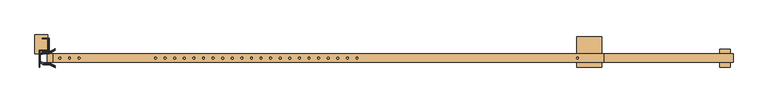
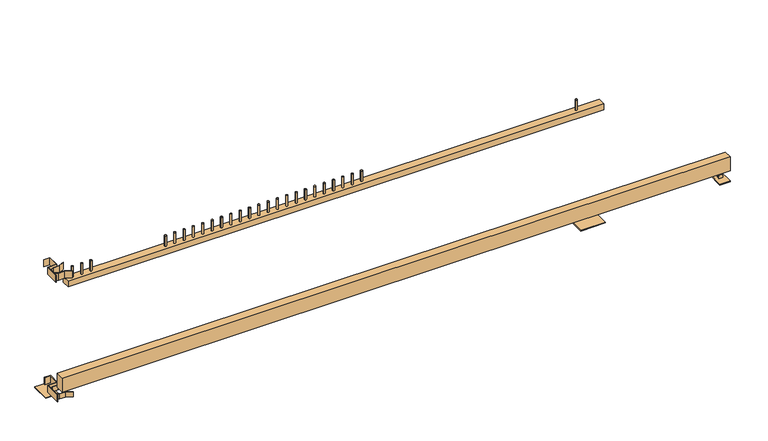
"""IFC4 building model written with IfcOpenShell, lengths in millimetres: door geometry, NLRS_90_DO_UN_schuifpoort met spijlen_gen_rsf : schuifpoort automatisch bxh 7000x1800-NP."""

import ifcopenshell
import ifcopenshell.guid

model = None  # the IFC model being written
_history = None  # IfcOwnerHistory: only IFC2X3 demands one
_inside = {}  # id of a spatial element -> (the spatial element, [elements in it])
_under = {}  # id of a project, library or spatial element -> (it, [spatial elements below it])
_declared = {}  # id of a project -> (the project, [libraries it declares])
_typed = {}  # id of a type object -> (the type object, [elements of that type])
_made_of = {}  # id of a material, layer set ... -> (it, [elements and type objects made of it])


def new_model(schema):
    """Start an empty IFC model of exactly this schema.

    Asked for "IFC4X3", IfcOpenShell would pick the latest addendum, in which some entities
    have other attributes; the version numbers below select the first issue.
    IFC2X3 requires an IfcOwnerHistory on every rooted entity: one is made here for all.
    """
    global model, _history
    if schema == "IFC4X3":
        model = ifcopenshell.file(schema_version=(4, 3, 0, 0))
    else:
        model = ifcopenshell.file(schema=schema)
    _inside.clear()
    _under.clear()
    _declared.clear()
    _typed.clear()
    _made_of.clear()
    _history = None
    if model.schema == "IFC2X3":
        org = make("IfcOrganization", Name="unknown")
        user = make(
            "IfcPersonAndOrganization",
            ThePerson=make("IfcPerson", FamilyName="unknown"),
            TheOrganization=org,
        )
        app = make(
            "IfcApplication",
            ApplicationDeveloper=org,
            Version="unknown",
            ApplicationFullName="unknown",
            ApplicationIdentifier="unknown",
        )
        _history = make(
            "IfcOwnerHistory",
            OwningUser=user,
            OwningApplication=app,
            ChangeAction="ADDED",
            CreationDate=0,
        )
    return model


def make(cls, **values):
    """One entity of the class cls with the attributes given. An attribute that is None is left unset."""
    return model.create_entity(
        cls, **{name: value for name, value in values.items() if value is not None}
    )


def rooted(cls, **values):
    """An entity with a GlobalId (a new one), such as an element, a storey or a relation."""
    return make(cls, GlobalId=ifcopenshell.guid.new(), OwnerHistory=_history, **values)


def si_unit(unit_type, name, prefix=None):
    """IfcSIUnit, for example si_unit("LENGTHUNIT", "METRE", prefix="MILLI")."""
    return make("IfcSIUnit", UnitType=unit_type, Prefix=prefix, Name=name)


def assignment(units):
    """IfcUnitAssignment: the units of a project."""
    return None if units is None else make("IfcUnitAssignment", Units=units)


def point(xyz):
    """IfcCartesianPoint."""
    return None if xyz is None else make("IfcCartesianPoint", Coordinates=xyz)


def direction(xyz):
    """IfcDirection."""
    return None if xyz is None else make("IfcDirection", DirectionRatios=xyz)


def frame(location, z_axis=None, x_axis=None):
    """IfcAxis2Placement3D, a coordinate frame: its origin and axes. An axis left out is left unset."""
    return make(
        "IfcAxis2Placement3D",
        Location=point(location),
        Axis=direction(z_axis),
        RefDirection=direction(x_axis),
    )


def frame_2d(location, x_axis=None):
    """IfcAxis2Placement2D, a coordinate frame in the plane: its origin and x axis."""
    return make(
        "IfcAxis2Placement2D", Location=point(location), RefDirection=direction(x_axis)
    )


def origin():
    """The frame at (0, 0, 0) with its axes left unset."""
    return frame((0.0, 0.0, 0.0))


def origin_with_axes():
    """The frame at (0, 0, 0) with the z axis (0, 0, 1) and the x axis (1, 0, 0) written out."""
    return frame((0.0, 0.0, 0.0), z_axis=(0.0, 0.0, 1.0), x_axis=(1.0, 0.0, 0.0))


def place(relative_to, where):
    """IfcLocalPlacement: puts the frame where relative to a parent placement (None: the world)."""
    return make(
        "IfcLocalPlacement", PlacementRelTo=relative_to, RelativePlacement=where
    )


def context(
    kind, dimensions, precision=None, world=None, true_north=None, identifier=None
):
    """IfcGeometricRepresentationContext, for example the 3D "Model" context."""
    return make(
        "IfcGeometricRepresentationContext",
        ContextIdentifier=identifier,
        ContextType=kind,
        CoordinateSpaceDimension=dimensions,
        Precision=precision,
        WorldCoordinateSystem=world,
        TrueNorth=true_north,
    )


def project(units=None, contexts=None):
    """IfcProject with its units and contexts."""
    return rooted(
        "IfcProject",
        Name="project",
        RepresentationContexts=contexts,
        UnitsInContext=assignment(units),
    )


def spatial(cls, under=None, at=None, **own):
    """A site, building, storey or space (cls), placed at a placement, below another one or the project."""
    s = rooted(cls, ObjectPlacement=at, **own)
    if under is not None:
        _under.setdefault(under.id(), (under, []))[1].append(s)
    return s


def polyline(points):
    """IfcPolyline through the points."""
    return make("IfcPolyline", Points=[point(p) for p in points])


def circle_curve(where, radius):
    """IfcCircle in the frame where."""
    return make("IfcCircle", Position=where, Radius=radius)


def trimmed(basis, trim1, trim2, sense, master):
    """IfcTrimmedCurve: the piece of a basis curve between two trims."""
    return make(
        "IfcTrimmedCurve",
        BasisCurve=basis,
        Trim1=trim1,
        Trim2=trim2,
        SenseAgreement=sense,
        MasterRepresentation=master,
    )


def segment(curve, same_sense, transition):
    """IfcCompositeCurveSegment."""
    return make(
        "IfcCompositeCurveSegment",
        Transition=transition,
        SameSense=same_sense,
        ParentCurve=curve,
    )


def composite_curve(segments, self_intersect=None):
    """IfcCompositeCurve: segments joined end to end."""
    return make("IfcCompositeCurve", Segments=segments, SelfIntersect=self_intersect)


def outline(outer, holes=None, kind="AREA"):
    """IfcArbitraryClosedProfileDef: a profile drawn as a closed curve; with holes, ...WithVoids."""
    if holes is None:
        return make("IfcArbitraryClosedProfileDef", ProfileType=kind, OuterCurve=outer)
    return make(
        "IfcArbitraryProfileDefWithVoids",
        ProfileType=kind,
        OuterCurve=outer,
        InnerCurves=holes,
    )


def extrude(swept, where, along, depth):
    """IfcExtrudedAreaSolid: the profile swept, set in the frame where, extruded along a direction by depth."""
    return make(
        "IfcExtrudedAreaSolid",
        SweptArea=swept,
        Position=where,
        ExtrudedDirection=direction(along),
        Depth=depth,
    )


def shape(context_of_items, identifier, shape_type, items):
    """IfcShapeRepresentation: the items that make up one representation, for example the "Body"."""
    return make(
        "IfcShapeRepresentation",
        ContextOfItems=context_of_items,
        RepresentationIdentifier=identifier,
        RepresentationType=shape_type,
        Items=items,
    )


def source(mapping_origin, context_of_items, identifier, shape_type, items):
    """IfcRepresentationMap: a shape defined once, which mapped items show again and again."""
    return make(
        "IfcRepresentationMap",
        MappingOrigin=mapping_origin,
        MappedRepresentation=shape(context_of_items, identifier, shape_type, items),
    )


def transform(
    local_origin,
    x_axis=None,
    y_axis=None,
    z_axis=None,
    scale=None,
    scale2=None,
    scale3=None,
    uniform=True,
):
    """IfcCartesianTransformationOperator3D, or its non-uniform kind. x_axis, y_axis, z_axis: its Axis1, 2, 3."""
    if uniform:
        return make(
            "IfcCartesianTransformationOperator3D",
            Axis1=direction(x_axis),
            Axis2=direction(y_axis),
            LocalOrigin=point(local_origin),
            Scale=scale,
            Axis3=direction(z_axis),
        )
    return make(
        "IfcCartesianTransformationOperator3DnonUniform",
        Axis1=direction(x_axis),
        Axis2=direction(y_axis),
        LocalOrigin=point(local_origin),
        Scale=scale,
        Axis3=direction(z_axis),
        Scale2=scale2,
        Scale3=scale3,
    )


def mapped(mapping_source, mapping_target):
    """IfcMappedItem: shows the shape of a source again, moved by a transform."""
    return make(
        "IfcMappedItem", MappingSource=mapping_source, MappingTarget=mapping_target
    )


def made_of(thing, what):
    """Note that an element or type object is made of a material, layer set ...; save() writes the relation."""
    if what is not None:
        _made_of.setdefault(what.id(), (what, []))[1].append(thing)
    return thing


def element(
    cls,
    number,
    at=None,
    inside=None,
    cuts=None,
    type_object=None,
    material=None,
    context=None,
    identifier="Body",
    shape_type=None,
    held_by="IfcProductDefinitionShape",
    body=None,
    shapes=None,
    **own,
):
    """One element of the class cls, such as IfcWall. Its Tag is "e" and its number.

    at: its placement. inside: the storey or other place that contains it. cuts: it is an
    opening in that element (IfcRelVoidsElement). A single representation is given by context,
    identifier, shape_type and body (its items); several are given by shapes. held_by: the class
    of the entity that holds the representations. save() writes the other relations.
    """
    e = rooted(cls, Tag="e%d" % number, ObjectPlacement=at, **own)
    if body is not None:
        shapes = [shape(context, identifier, shape_type, body)]
    if shapes is not None:
        e.Representation = make(held_by, Representations=shapes)
    if inside is not None:
        _inside.setdefault(inside.id(), (inside, []))[1].append(e)
    if cuts is not None:
        rooted(
            "IfcRelVoidsElement", RelatingBuildingElement=cuts, RelatedOpeningElement=e
        )
    if type_object is not None:
        _typed.setdefault(type_object.id(), (type_object, []))[1].append(e)
    return made_of(e, material)


def aggregate(whole, parts):
    """IfcRelAggregates: a whole, such as a stair, and the parts it consists of."""
    return rooted("IfcRelAggregates", RelatingObject=whole, RelatedObjects=parts)


def save(model, path):
    """Write the relations noted so far, then the file.

    IfcRelAggregates (storeys below a building ...), IfcRelContainedInSpatialStructure (elements
    in a storey), IfcRelDefinesByType, IfcRelAssociatesMaterial and IfcRelDeclares: one each for
    every whole, place, type object, material and project.
    """
    for whole, parts in _under.values():
        aggregate(whole, parts)
    for where, things in _inside.values():
        rooted(
            "IfcRelContainedInSpatialStructure",
            RelatedElements=things,
            RelatingStructure=where,
        )
    for kind, things in _typed.values():
        rooted("IfcRelDefinesByType", RelatedObjects=things, RelatingType=kind)
    for what, things in _made_of.values():
        rooted("IfcRelAssociatesMaterial", RelatedObjects=things, RelatingMaterial=what)
    for by, libraries in _declared.values():
        rooted("IfcRelDeclares", RelatingContext=by, RelatedDefinitions=libraries)
    model.write(path)


def door_84a52a24(model_context):
    return source(origin(), model_context, "Body", "SweptSolid", [
        extrude(outline(composite_curve([segment(trimmed(circle_curve(frame_2d((-3115.5, 0.0)), 12.5), [point((-3103.0, 0.0))], [point((-3128.0, 0.0))], False, "CARTESIAN"), True, "CONTINUOUS"), segment(trimmed(circle_curve(frame_2d((-3115.5, 0.0)), 12.5), [point((-3128.0, 0.0))], [point((-3103.0, 0.0))], False, "CARTESIAN"), True, "CONTINUOUS")], self_intersect=False)), frame((0.0, 0.0, 1650.0), z_axis=(0.0, 0.0, 1.0), x_axis=(1.0, 0.0, 0.0)), (0.0, 0.0, 1.0), 150.0),
        extrude(outline(composite_curve([segment(trimmed(circle_curve(frame_2d((-3241.5, 0.0)), 12.5), [point((-3229.0, 0.0))], [point((-3254.0, 0.0))], False, "CARTESIAN"), True, "CONTINUOUS"), segment(trimmed(circle_curve(frame_2d((-3241.5, 0.0)), 12.5), [point((-3254.0, 0.0))], [point((-3229.0, 0.0))], False, "CARTESIAN"), True, "CONTINUOUS")], self_intersect=False)), frame((0.0, 0.0, 1650.0), z_axis=(0.0, 0.0, 1.0), x_axis=(1.0, 0.0, 0.0)), (0.0, 0.0, 1.0), 150.0),
        extrude(outline(composite_curve([segment(trimmed(circle_curve(frame_2d((-3367.5, 0.0)), 12.5), [point((-3355.0, 0.0))], [point((-3380.0, 0.0))], False, "CARTESIAN"), True, "CONTINUOUS"), segment(trimmed(circle_curve(frame_2d((-3367.5, 0.0)), 12.5), [point((-3380.0, 0.0))], [point((-3355.0, 0.0))], False, "CARTESIAN"), True, "CONTINUOUS")], self_intersect=False)), frame((0.0, 0.0, 1650.0), z_axis=(0.0, 0.0, 1.0), x_axis=(1.0, 0.0, 0.0)), (0.0, 0.0, 1.0), 150.0),
        extrude(outline(polyline([(3745.0, 280.5), (3745.0, -119.5), (3415.0, -119.5), (3415.0, 280.5), (3745.0, 280.5)])), origin_with_axes(), (0.0, 0.0, 1.0), 12.0),
        extrude(outline(composite_curve([segment(trimmed(circle_curve(frame_2d((3424.5, 0.0)), 12.5), [point((3437.0, 0.0))], [point((3412.0, 0.0))], False, "CARTESIAN"), True, "CONTINUOUS"), segment(trimmed(circle_curve(frame_2d((3424.5, 0.0)), 12.5), [point((3412.0, 0.0))], [point((3437.0, 0.0))], False, "CARTESIAN"), True, "CONTINUOUS")], self_intersect=False)), frame((0.0, 0.0, 1650.0), z_axis=(0.0, 0.0, 1.0), x_axis=(1.0, 0.0, 0.0)), (0.0, 0.0, 1.0), 150.0),
        extrude(outline(composite_curve([segment(trimmed(circle_curve(frame_2d((-727.5, 0.0)), 12.5), [point((-715.0, 0.0))], [point((-740.0, 0.0))], False, "CARTESIAN"), True, "CONTINUOUS"), segment(trimmed(circle_curve(frame_2d((-727.5, 0.0)), 12.5), [point((-740.0, 0.0))], [point((-715.0, 0.0))], False, "CARTESIAN"), True, "CONTINUOUS")], self_intersect=False)), frame((0.0, 0.0, 1650.0), z_axis=(0.0, 0.0, 1.0), x_axis=(1.0, 0.0, 0.0)), (0.0, 0.0, 1.0), 150.0),
        extrude(outline(composite_curve([segment(trimmed(circle_curve(frame_2d((-2111.5, 0.0)), 12.5), [point((-2099.0, 0.0))], [point((-2124.0, 0.0))], False, "CARTESIAN"), True, "CONTINUOUS"), segment(trimmed(circle_curve(frame_2d((-2111.5, 0.0)), 12.5), [point((-2124.0, 0.0))], [point((-2099.0, 0.0))], False, "CARTESIAN"), True, "CONTINUOUS")], self_intersect=False)), frame((0.0, 0.0, 1650.0), z_axis=(0.0, 0.0, 1.0), x_axis=(1.0, 0.0, 0.0)), (0.0, 0.0, 1.0), 150.0),
        extrude(outline(composite_curve([segment(trimmed(circle_curve(frame_2d((531.5, 0.0)), 12.5), [point((544.0, 0.0))], [point((519.0, 0.0))], False, "CARTESIAN"), True, "CONTINUOUS"), segment(trimmed(circle_curve(frame_2d((531.5, 0.0)), 12.5), [point((519.0, 0.0))], [point((544.0, 0.0))], False, "CARTESIAN"), True, "CONTINUOUS")], self_intersect=False)), frame((0.0, 0.0, 1650.0), z_axis=(0.0, 0.0, 1.0), x_axis=(1.0, 0.0, 0.0)), (0.0, 0.0, 1.0), 150.0),
        extrude(outline(composite_curve([segment(trimmed(circle_curve(frame_2d((405.5, 0.0)), 12.5), [point((418.0, 0.0))], [point((393.0, 0.0))], False, "CARTESIAN"), True, "CONTINUOUS"), segment(trimmed(circle_curve(frame_2d((405.5, 0.0)), 12.5), [point((393.0, 0.0))], [point((418.0, 0.0))], False, "CARTESIAN"), True, "CONTINUOUS")], self_intersect=False)), frame((0.0, 0.0, 1650.0), z_axis=(0.0, 0.0, 1.0), x_axis=(1.0, 0.0, 0.0)), (0.0, 0.0, 1.0), 150.0),
        extrude(outline(composite_curve([segment(trimmed(circle_curve(frame_2d((279.5, 0.0)), 12.5), [point((292.0, 0.0))], [point((267.0, 0.0))], False, "CARTESIAN"), True, "CONTINUOUS"), segment(trimmed(circle_curve(frame_2d((279.5, 0.0)), 12.5), [point((267.0, 0.0))], [point((292.0, 0.0))], False, "CARTESIAN"), True, "CONTINUOUS")], self_intersect=False)), frame((0.0, 0.0, 1650.0), z_axis=(0.0, 0.0, 1.0), x_axis=(1.0, 0.0, 0.0)), (0.0, 0.0, 1.0), 150.0),
        extrude(outline(composite_curve([segment(trimmed(circle_curve(frame_2d((153.5, 0.0)), 12.5), [point((166.0, 0.0))], [point((141.0, 0.0))], False, "CARTESIAN"), True, "CONTINUOUS"), segment(trimmed(circle_curve(frame_2d((153.5, 0.0)), 12.5), [point((141.0, 0.0))], [point((166.0, 0.0))], False, "CARTESIAN"), True, "CONTINUOUS")], self_intersect=False)), frame((0.0, 0.0, 1650.0), z_axis=(0.0, 0.0, 1.0), x_axis=(1.0, 0.0, 0.0)), (0.0, 0.0, 1.0), 150.0),
        extrude(outline(composite_curve([segment(trimmed(circle_curve(frame_2d((27.5, 0.0)), 12.5), [point((40.0, 0.0))], [point((15.0, 0.0))], False, "CARTESIAN"), True, "CONTINUOUS"), segment(trimmed(circle_curve(frame_2d((27.5, 0.0)), 12.5), [point((15.0, 0.0))], [point((40.0, 0.0))], False, "CARTESIAN"), True, "CONTINUOUS")], self_intersect=False)), frame((0.0, 0.0, 1650.0), z_axis=(0.0, 0.0, 1.0), x_axis=(1.0, 0.0, 0.0)), (0.0, 0.0, 1.0), 150.0),
        extrude(outline(composite_curve([segment(trimmed(circle_curve(frame_2d((-98.5, 0.0)), 12.5), [point((-86.0, 0.0))], [point((-111.0, 0.0))], False, "CARTESIAN"), True, "CONTINUOUS"), segment(trimmed(circle_curve(frame_2d((-98.5, 0.0)), 12.5), [point((-111.0, 0.0))], [point((-86.0, 0.0))], False, "CARTESIAN"), True, "CONTINUOUS")], self_intersect=False)), frame((0.0, 0.0, 1650.0), z_axis=(0.0, 0.0, 1.0), x_axis=(1.0, 0.0, 0.0)), (0.0, 0.0, 1.0), 150.0),
        extrude(outline(composite_curve([segment(trimmed(circle_curve(frame_2d((-224.5, 0.0)), 12.5), [point((-212.0, 0.0))], [point((-237.0, 0.0))], False, "CARTESIAN"), True, "CONTINUOUS"), segment(trimmed(circle_curve(frame_2d((-224.5, 0.0)), 12.5), [point((-237.0, 0.0))], [point((-212.0, 0.0))], False, "CARTESIAN"), True, "CONTINUOUS")], self_intersect=False)), frame((0.0, 0.0, 1650.0), z_axis=(0.0, 0.0, 1.0), x_axis=(1.0, 0.0, 0.0)), (0.0, 0.0, 1.0), 150.0),
        extrude(outline(composite_curve([segment(trimmed(circle_curve(frame_2d((-350.5, 0.0)), 12.5), [point((-338.0, 0.0))], [point((-363.0, 0.0))], False, "CARTESIAN"), True, "CONTINUOUS"), segment(trimmed(circle_curve(frame_2d((-350.5, 0.0)), 12.5), [point((-363.0, 0.0))], [point((-338.0, 0.0))], False, "CARTESIAN"), True, "CONTINUOUS")], self_intersect=False)), frame((0.0, 0.0, 1650.0), z_axis=(0.0, 0.0, 1.0), x_axis=(1.0, 0.0, 0.0)), (0.0, 0.0, 1.0), 150.0),
        extrude(outline(composite_curve([segment(trimmed(circle_curve(frame_2d((-476.5, 0.0)), 12.5), [point((-464.0, 0.0))], [point((-489.0, 0.0))], False, "CARTESIAN"), True, "CONTINUOUS"), segment(trimmed(circle_curve(frame_2d((-476.5, 0.0)), 12.5), [point((-489.0, 0.0))], [point((-464.0, 0.0))], False, "CARTESIAN"), True, "CONTINUOUS")], self_intersect=False)), frame((0.0, 0.0, 1650.0), z_axis=(0.0, 0.0, 1.0), x_axis=(1.0, 0.0, 0.0)), (0.0, 0.0, 1.0), 150.0),
        extrude(outline(composite_curve([segment(trimmed(circle_curve(frame_2d((-602.5, 0.0)), 12.5), [point((-590.0, 0.0))], [point((-615.0, 0.0))], False, "CARTESIAN"), True, "CONTINUOUS"), segment(trimmed(circle_curve(frame_2d((-602.5, 0.0)), 12.5), [point((-615.0, 0.0))], [point((-590.0, 0.0))], False, "CARTESIAN"), True, "CONTINUOUS")], self_intersect=False)), frame((0.0, 0.0, 1650.0), z_axis=(0.0, 0.0, 1.0), x_axis=(1.0, 0.0, 0.0)), (0.0, 0.0, 1.0), 150.0),
        extrude(outline(composite_curve([segment(trimmed(circle_curve(frame_2d((-852.5, 0.0)), 12.5), [point((-840.0, 0.0))], [point((-865.0, 0.0))], False, "CARTESIAN"), True, "CONTINUOUS"), segment(trimmed(circle_curve(frame_2d((-852.5, 0.0)), 12.5), [point((-865.0, 0.0))], [point((-840.0, 0.0))], False, "CARTESIAN"), True, "CONTINUOUS")], self_intersect=False)), frame((0.0, 0.0, 1650.0), z_axis=(0.0, 0.0, 1.0), x_axis=(1.0, 0.0, 0.0)), (0.0, 0.0, 1.0), 150.0),
        extrude(outline(composite_curve([segment(trimmed(circle_curve(frame_2d((-978.5, 0.0)), 12.5), [point((-966.0, 0.0))], [point((-991.0, 0.0))], False, "CARTESIAN"), True, "CONTINUOUS"), segment(trimmed(circle_curve(frame_2d((-978.5, 0.0)), 12.5), [point((-991.0, 0.0))], [point((-966.0, 0.0))], False, "CARTESIAN"), True, "CONTINUOUS")], self_intersect=False)), frame((0.0, 0.0, 1650.0), z_axis=(0.0, 0.0, 1.0), x_axis=(1.0, 0.0, 0.0)), (0.0, 0.0, 1.0), 150.0),
        extrude(outline(composite_curve([segment(trimmed(circle_curve(frame_2d((-1104.5, 0.0)), 12.5), [point((-1092.0, 0.0))], [point((-1117.0, 0.0))], False, "CARTESIAN"), True, "CONTINUOUS"), segment(trimmed(circle_curve(frame_2d((-1104.5, 0.0)), 12.5), [point((-1117.0, 0.0))], [point((-1092.0, 0.0))], False, "CARTESIAN"), True, "CONTINUOUS")], self_intersect=False)), frame((0.0, 0.0, 1650.0), z_axis=(0.0, 0.0, 1.0), x_axis=(1.0, 0.0, 0.0)), (0.0, 0.0, 1.0), 150.0),
        extrude(outline(composite_curve([segment(trimmed(circle_curve(frame_2d((-1230.5, 0.0)), 12.5), [point((-1218.0, 0.0))], [point((-1243.0, 0.0))], False, "CARTESIAN"), True, "CONTINUOUS"), segment(trimmed(circle_curve(frame_2d((-1230.5, 0.0)), 12.5), [point((-1243.0, 0.0))], [point((-1218.0, 0.0))], False, "CARTESIAN"), True, "CONTINUOUS")], self_intersect=False)), frame((0.0, 0.0, 1650.0), z_axis=(0.0, 0.0, 1.0), x_axis=(1.0, 0.0, 0.0)), (0.0, 0.0, 1.0), 150.0),
        extrude(outline(composite_curve([segment(trimmed(circle_curve(frame_2d((-1356.5, 0.0)), 12.5), [point((-1344.0, 0.0))], [point((-1369.0, 0.0))], False, "CARTESIAN"), True, "CONTINUOUS"), segment(trimmed(circle_curve(frame_2d((-1356.5, 0.0)), 12.5), [point((-1369.0, 0.0))], [point((-1344.0, 0.0))], False, "CARTESIAN"), True, "CONTINUOUS")], self_intersect=False)), frame((0.0, 0.0, 1650.0), z_axis=(0.0, 0.0, 1.0), x_axis=(1.0, 0.0, 0.0)), (0.0, 0.0, 1.0), 150.0),
        extrude(outline(composite_curve([segment(trimmed(circle_curve(frame_2d((-1482.5, 0.0)), 12.5), [point((-1470.0, 0.0))], [point((-1495.0, 0.0))], False, "CARTESIAN"), True, "CONTINUOUS"), segment(trimmed(circle_curve(frame_2d((-1482.5, 0.0)), 12.5), [point((-1495.0, 0.0))], [point((-1470.0, 0.0))], False, "CARTESIAN"), True, "CONTINUOUS")], self_intersect=False)), frame((0.0, 0.0, 1650.0), z_axis=(0.0, 0.0, 1.0), x_axis=(1.0, 0.0, 0.0)), (0.0, 0.0, 1.0), 150.0),
        extrude(outline(composite_curve([segment(trimmed(circle_curve(frame_2d((-1608.5, 0.0)), 12.5), [point((-1596.0, 0.0))], [point((-1621.0, 0.0))], False, "CARTESIAN"), True, "CONTINUOUS"), segment(trimmed(circle_curve(frame_2d((-1608.5, 0.0)), 12.5), [point((-1621.0, 0.0))], [point((-1596.0, 0.0))], False, "CARTESIAN"), True, "CONTINUOUS")], self_intersect=False)), frame((0.0, 0.0, 1650.0), z_axis=(0.0, 0.0, 1.0), x_axis=(1.0, 0.0, 0.0)), (0.0, 0.0, 1.0), 150.0),
        extrude(outline(composite_curve([segment(trimmed(circle_curve(frame_2d((-1734.5, 0.0)), 12.5), [point((-1722.0, 0.0))], [point((-1747.0, 0.0))], False, "CARTESIAN"), True, "CONTINUOUS"), segment(trimmed(circle_curve(frame_2d((-1734.5, 0.0)), 12.5), [point((-1747.0, 0.0))], [point((-1722.0, 0.0))], False, "CARTESIAN"), True, "CONTINUOUS")], self_intersect=False)), frame((0.0, 0.0, 1650.0), z_axis=(0.0, 0.0, 1.0), x_axis=(1.0, 0.0, 0.0)), (0.0, 0.0, 1.0), 150.0),
        extrude(outline(composite_curve([segment(trimmed(circle_curve(frame_2d((-1860.5, 0.0)), 12.5), [point((-1848.0, 0.0))], [point((-1873.0, 0.0))], False, "CARTESIAN"), True, "CONTINUOUS"), segment(trimmed(circle_curve(frame_2d((-1860.5, 0.0)), 12.5), [point((-1873.0, 0.0))], [point((-1848.0, 0.0))], False, "CARTESIAN"), True, "CONTINUOUS")], self_intersect=False)), frame((0.0, 0.0, 1650.0), z_axis=(0.0, 0.0, 1.0), x_axis=(1.0, 0.0, 0.0)), (0.0, 0.0, 1.0), 150.0),
        extrude(outline(composite_curve([segment(trimmed(circle_curve(frame_2d((-1986.5, 0.0)), 12.5), [point((-1974.0, 0.0))], [point((-1999.0, 0.0))], False, "CARTESIAN"), True, "CONTINUOUS"), segment(trimmed(circle_curve(frame_2d((-1986.5, 0.0)), 12.5), [point((-1999.0, 0.0))], [point((-1974.0, 0.0))], False, "CARTESIAN"), True, "CONTINUOUS")], self_intersect=False)), frame((0.0, 0.0, 1650.0), z_axis=(0.0, 0.0, 1.0), x_axis=(1.0, 0.0, 0.0)), (0.0, 0.0, 1.0), 150.0),
        extrude(outline(polyline([(-3430.0, -104.7285156), (-3510.75, -63.3066406), (-3586.53125, -63.3066406), (-3633.0, -39.4667969), (-3633.0, 39.4707031), (-3586.53125, 63.3105469), (-3510.75, 63.3105469), (-3430.0, 104.7324219), (-3428.15625, 101.1738281), (-3509.78125, 59.3105469), (-3585.5625, 59.3105469), (-3629.0, 37.0332031), (-3629.0, -37.0292969), (-3585.5625, -59.3066406), (-3509.78125, -59.3066406), (-3428.15625, -101.1699219), (-3430.0, -104.7285156)])), frame((0.0, 0.0, 1720.0), z_axis=(0.0, 0.0, 1.0), x_axis=(1.0, 0.0, 0.0)), (0.0, 0.0, 1.0), 100.0),
        extrude(outline(polyline([(-3638.0, 105.534128), (-3524.015625, 105.534128), (-3524.015625, 255.534128), (-3601.25, 255.534128), (-3601.25, 260.534128), (-3519.015625, 260.534128), (-3519.015625, 100.534128), (-3633.0, 100.534128), (-3633.0, -85.4980469), (-3638.0, -85.4980469), (-3638.0, 105.534128)])), frame((0.0, 0.0, 1720.0), z_axis=(0.0, 0.0, 1.0), x_axis=(1.0, 0.0, 0.0)), (0.0, 0.0, 1.0), 100.0),
        extrude(outline(composite_curve([segment(polyline([(12.0, 5337.0), (12.0, 5387.0), (42.0, 5387.0)]), True, "CONTINUOUS"), segment(trimmed(circle_curve(frame_2d((42.0, 5362.0)), 25.0), [point((42.0, 5387.0))], [point((42.0, 5337.0))], False, "CARTESIAN"), True, "CONTINUOUS"), segment(polyline([(42.0, 5337.0), (12.0, 5337.0)]), True, "CONTINUOUS")], self_intersect=False)), frame((0.0, 11.0, 0.0), z_axis=(0.0, 1.0, 0.0), x_axis=(0.0, 0.0, 1.0)), (0.0, 0.0, 1.0), 8.0),
        extrude(outline(composite_curve([segment(polyline([(12.0, 5337.0), (12.0, 5387.0), (42.0, 5387.0)]), True, "CONTINUOUS"), segment(trimmed(circle_curve(frame_2d((42.0, 5362.0)), 25.0), [point((42.0, 5387.0))], [point((42.0, 5337.0))], False, "CARTESIAN"), True, "CONTINUOUS"), segment(polyline([(42.0, 5337.0), (12.0, 5337.0)]), True, "CONTINUOUS")], self_intersect=False)), frame((0.0, -19.0, 0.0), z_axis=(0.0, 1.0, 0.0), x_axis=(0.0, 0.0, 1.0)), (0.0, 0.0, 1.0), 8.0),
        extrude(outline(polyline([(5432.0, 120.0), (5432.0, -120.0), (5292.0, -120.0), (5292.0, 120.0), (5432.0, 120.0)])), origin_with_axes(), (0.0, 0.0, 1.0), 12.0),
        extrude(outline(polyline([(5372.0, 11.0), (5372.0, -11.0), (5352.0, -11.0), (5352.0, 11.0), (5372.0, 11.0)])), frame((0.0, 0.0, 12.0), z_axis=(0.0, 0.0, 1.0), x_axis=(1.0, 0.0, 0.0)), (0.0, 0.0, 1.0), 88.0),
        extrude(outline(polyline([(-3429.5, -126.125), (-3509.75, -84.8125), (-3585.75, -84.8125), (-3633.0, -60.585938), (-3633.0, 60.585938), (-3585.75, 84.8125), (-3509.75, 84.8125), (-3429.5, 126.125), (-3427.2114608, 121.6794867), (-3508.5385575, 79.8125), (-3584.542883, 79.8125), (-3628.0, 57.5306685), (-3628.0, -57.5306685), (-3584.542883, -79.8125), (-3508.5385575, -79.8125), (-3427.2114608, -121.6794867), (-3429.5, -126.125)])), frame((0.0, 0.0, 39.0), z_axis=(0.0, 0.0, 1.0), x_axis=(1.0, 0.0, 0.0)), (0.0, 0.0, 1.0), 70.0),
        extrude(outline(polyline([(-3638.0, 105.5), (-3515.0, 105.5), (-3515.0, 255.5), (-3593.0, 255.5), (-3593.0, 260.5), (-3510.0, 260.5), (-3510.0, 100.5), (-3633.0, 100.5), (-3633.0, -119.5), (-3638.0, -119.5), (-3638.0, 105.5)])), frame((0.0, 0.0, 39.0), z_axis=(0.0, 0.0, 1.0), x_axis=(1.0, 0.0, 0.0)), (0.0, 0.0, 1.0), 100.0),
        extrude(outline(polyline([(5467.0, 55.0), (5467.0, -55.0), (-3535.5, -55.0), (-3535.5, 55.0), (5467.0, 55.0)])), frame((0.0, 0.0, 100.0), z_axis=(0.0, 0.0, 1.0), x_axis=(1.0, 0.0, 0.0)), (0.0, 0.0, 1.0), 200.0),
        extrude(outline(polyline([(-3525.0, 305.0), (-3525.0, 55.0), (-3695.0, 55.0), (-3695.0, 305.0), (-3525.0, 305.0)])), origin_with_axes(), (0.0, 0.0, 1.0), 12.0),
        extrude(outline(polyline([(3767.5, 55.0), (3767.5, -55.0), (-3455.5, -55.0), (-3455.5, 55.0), (3767.5, 55.0)])), frame((0.0, 0.0, 1570.0), z_axis=(0.0, 0.0, 1.0), x_axis=(1.0, 0.0, 0.0)), (0.0, 0.0, 1.0), 80.0),
    ])


if __name__ == "__main__":
    model = new_model("IFC4")
    model_context = context("Model", 3, world=origin())
    ifc_project = project(units=[si_unit("LENGTHUNIT", "METRE", prefix="MILLI")], contexts=[model_context])
    site = spatial("IfcSite", under=ifc_project)
    building = spatial("IfcBuilding", under=site)
    placement = place(None, origin())
    door_shape = door_84a52a24(model_context)
    element("IfcDoor", 1, ObjectType="NLRS_90_DO_UN_schuifpoort met spijlen_gen_rsf : schuifpoort automatisch bxh 7000x1800-NP", at=placement, inside=building, context=model_context, shape_type="MappedRepresentation", body=[
        mapped(door_shape, transform((0.0, 0.0, 0.0), x_axis=(1.0, 0.0, 0.0), y_axis=(0.0, 1.0, 0.0), z_axis=(0.0, 0.0, 1.0))),
    ])
    save(model, "model.ifc")

# Revit data of these elements
# Type "NLRS_90_DO_UN_schuifpoort met spijlen_gen_rsf : schuifpoort automatisch bxh 7000x1800-NP"
#   Type IFC Predefined Type = "GATE"
#   Export Type to IFC As = "IfcDoorType"
#   Type IfcGUID = "1A81voHkv98RYujw6ZYnX6"
#   IfcName[Type] = "schuifpoort automatisch bxh 7000x1800-NP"
#   IfcDescription[Type] = "schuifpoort doorgang bxh 7000x1800mm"
#   IfcExportAs[Type] = "IfcDoorType"
#   IfcExportType[Type] = "GATE"
#   NLRS_C_revit_versie = ""
#   NLRS_C_omschrijving_03 [instance default] = "doorgangsmaat"
#   NLRS_C_omschrijving_02 [instance default] = "stootplaat"
#   NLRS_C_omschrijving_01 [instance default] = "rolpoort"
#   NLRS_C_content_versie = ""
#   NLRS_C_content_provider = ""
#   NLRS_C_content_handleiding = ""
#   NLRS_C_content_datum_uitgifte = ""
#   NLRS_C_content_datum_gewijzigd = ""
#   NLRS_C_content_creator = ""
#   Model = "generiek"
#   Manufacturer = "Revit Standards Foundation"
#   Description = "schuifpoort doorgang bxh 7000x1800mm"
#   Assembly Code = "90.32"
#   NLRS_C_hoogte = 1800.00 mm
#   NLRS_C_breedte_03 = 7000.00 mm
#   NLRS_C_materiaal_02 = NLRS_n5_rubber_gen_bf
#   NLRS_C_materiaal_01 = NLRS_h4_aluminium 250-255-255_gen_rsf
#   URL = ""
#   Keynote = ""
#   Default Elevation = 0
# Element 1 (IfcDoor, "NLRS_90_DO_UN_schuifpoort met spijlen_gen_rsf : schuifpoort automatisch bxh 7000x1800-NP")
#   Materials on its faces: "NLRS_h4_aluminium 250-255-255_gen_rsf", "NLRS_n5_rubber_gen_bf"
# Materials
#   "NLRS_n5_rubber_gen_bf": class "N - Kunststoffen, rubbers", colour RGB 63 63 63, transparency 0, Keynote = "n5", Model = "generiek", Manufacturer = "Revit Standards Foundation", URL = "www.revitstandards.org", Description = "rubber daktegels 600x600mm", Cost = 0
#   "NLRS_h4_aluminium 250-255-255_gen_rsf": class "BCB class", colour RGB 250 255 255, transparency 0, Keynote = "h4", Model = "generiek", Manufacturer = "Revit Standards Foundation", URL = "www.revitstandards.org", Description = "aluminium wit", Cost = 0
